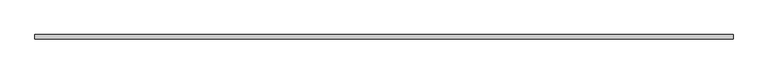
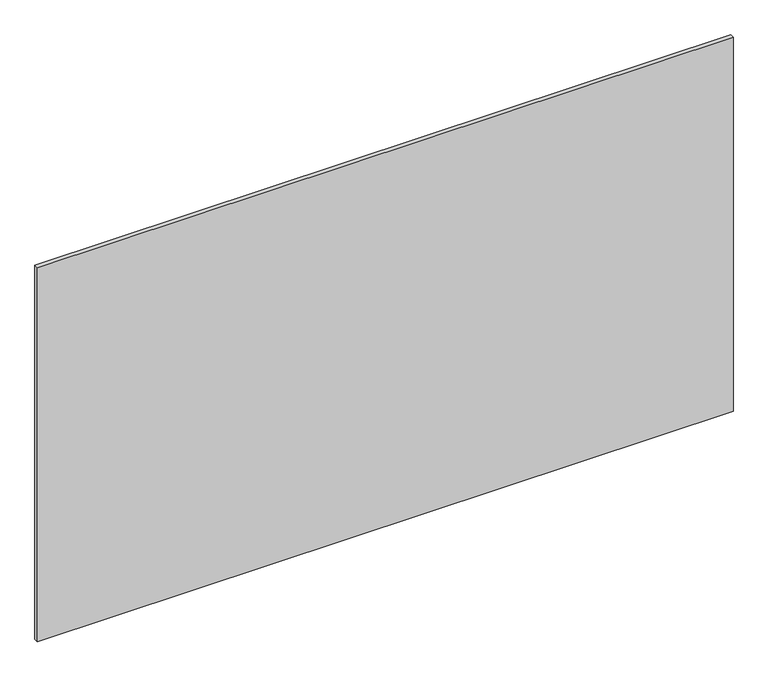
"""IFC4 building model written with IfcOpenShell, lengths in millimetres: railing geometry, ML_Painéis3 : ML_Painéis."""

from ifc_helpers import new_model, si_unit, frame, origin, place, context, project, spatial, polyline, outline, extrude, source, transform, mapped, element, save


def railing_0d959ca4(model_context):
    return source(origin(), model_context, "Body", "SweptSolid", [
        extrude(outline(polyline([(-4674.5702584, 2133.3602771), (-4674.5702584, 2121.3602771), (-6610.5702584, 2121.3602771), (-6610.5702584, 2133.3602771), (-4674.5702584, 2133.3602771)])), frame((0.0, 0.0, 4122.0679199), z_axis=(0.0, 0.0, 1.0), x_axis=(1.0, 0.0, 0.0)), (0.0, 0.0, 1.0), 1100.0),
    ])


if __name__ == "__main__":
    model = new_model("IFC4")
    model_context = context("Model", 3, world=origin())
    ifc_project = project(units=[si_unit("LENGTHUNIT", "METRE", prefix="MILLI")], contexts=[model_context])
    site = spatial("IfcSite", under=ifc_project)
    building = spatial("IfcBuilding", under=site)
    placement = place(None, origin())
    railing_shape = railing_0d959ca4(model_context)
    element("IfcRailing", 1, ObjectType="ML_Painéis3 : ML_Painéis", at=placement, inside=building, context=model_context, shape_type="MappedRepresentation", body=[
        mapped(railing_shape, transform((0.0, 0.0, 0.0), x_axis=(1.0, 0.0, 0.0), y_axis=(0.0, 1.0, 0.0), z_axis=(0.0, 0.0, 1.0))),
    ])
    save(model, "model.ifc")

# Revit data of these elements
# Type "ML_Painéis3 : ML_Painéis"
#   ME_Área [instance default] = 2.1296 m²
#   ME_Espessura [instance default] = 0.012 m
#   ME_Dist Painéis [instance default] = 0.002 m
#   ME_Compr Painéis [instance default] = 1.936 m
#   ME_Compr [instance default] = 1.94 m
#   ME_Altura [instance default] = 1.10 m
#   ME_Quant Painéis [instance default] = 3
#   ME_Painel Único [instance default] = yes
#   ME_Paineis Vários [instance default] = no
#   ME_Material Tipo Vidro [instance default] = .VIDRO GENÉRICO
# Element 1 (IfcRailing, "ML_Painéis3 : ML_Painéis")
#   Materials on its faces: ".VIDRO GENÉRICO"
# Materials
#   ".VIDRO GENÉRICO": class ".CC_VIDRO", colour RGB 0 128 192, transparency 0.9, Description = "Vidro comum", Cost = 0
